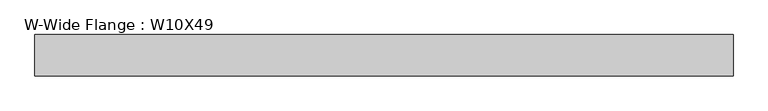
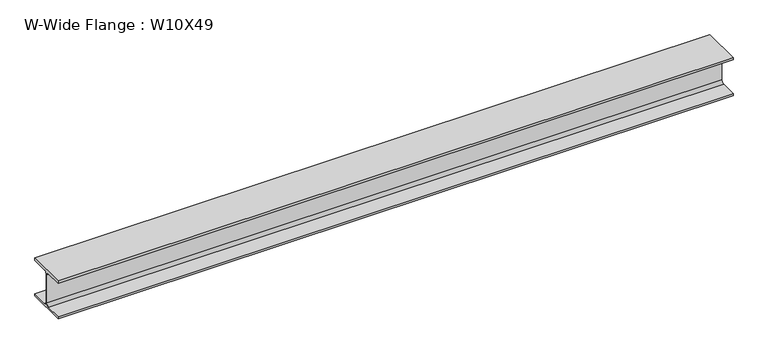
"""IFC4 building model written with IfcOpenShell, lengths in millimetres: beam geometry, W-Wide Flange : W10X49."""

from ifc_helpers import new_model, si_unit, point, frame, frame_2d, origin, place, context, project, spatial, polyline, circle_curve, trimmed, segment, composite_curve, outline, extrude, source, transform, mapped, element, save


def w_wide_flange_w10x49_85831f45(model_context):
    return source(origin(), model_context, "Body", "SweptSolid", [
        extrude(outline(composite_curve([segment(polyline([(127.0, -112.776), (127.0, -127.0), (-127.0, -127.0), (-127.0, -112.776), (-21.844, -112.776)]), True, "CONTINUOUS"), segment(trimmed(circle_curve(frame_2d((-21.844, -95.25)), 17.526), [point((-21.844, -112.776))], [point((-4.318, -95.25))], True, "CARTESIAN"), True, "CONTINUOUS"), segment(polyline([(-4.318, -95.25), (-4.318, 95.25)]), True, "CONTINUOUS"), segment(trimmed(circle_curve(frame_2d((-21.844, 95.25)), 17.526), [point((-4.318, 95.25))], [point((-21.844, 112.776))], True, "CARTESIAN"), True, "CONTINUOUS"), segment(polyline([(-21.844, 112.776), (-127.0, 112.776), (-127.0, 127.0), (127.0, 127.0), (127.0, 112.776), (21.844, 112.776)]), True, "CONTINUOUS"), segment(trimmed(circle_curve(frame_2d((21.844, 95.25)), 17.526), [point((21.844, 112.776))], [point((4.318, 95.25))], True, "CARTESIAN"), True, "CONTINUOUS"), segment(polyline([(4.318, 95.25), (4.318, -95.25)]), True, "CONTINUOUS"), segment(trimmed(circle_curve(frame_2d((21.844, -95.25)), 17.526), [point((4.318, -95.25))], [point((21.844, -112.776))], True, "CARTESIAN"), True, "CONTINUOUS"), segment(polyline([(21.844, -112.776), (127.0, -112.776)]), True, "CONTINUOUS")], self_intersect=False)), frame((-2142.7940989, 0.0, 0.0), z_axis=(1.0, 0.0, 0.0), x_axis=(0.0, 1.0, 0.0)), (0.0, 0.0, 1.0), 4286.3336069),
    ])


if __name__ == "__main__":
    model = new_model("IFC4")
    model_context = context("Model", 3, world=origin())
    ifc_project = project(units=[si_unit("LENGTHUNIT", "METRE", prefix="MILLI")], contexts=[model_context])
    site = spatial("IfcSite", under=ifc_project)
    building = spatial("IfcBuilding", under=site)
    placement = place(None, origin())
    w_wide_flange_w10x49_shape = w_wide_flange_w10x49_85831f45(model_context)
    element("IfcBeam", 1, ObjectType="W-Wide Flange : W10X49", at=placement, inside=building, context=model_context, shape_type="MappedRepresentation", body=[
        mapped(w_wide_flange_w10x49_shape, transform((0.0, 0.0, 0.0), x_axis=(1.0, 0.0, 0.0), y_axis=(0.0, 1.0, 0.0), z_axis=(0.0, 0.0, 1.0))),
    ])
    save(model, "model.ifc")

# Revit data of these elements
# Type "W-Wide Flange : W10X49"
#   Assembly Code = "B10"
#   W = 49
#   Length [instance default] = 1524 mm
#   bf = 254 mm
#   d = 254 mm
#   k = 31.75 mm
#   k2 = 17.526 mm
#   tf = 14.224 mm
#   tw = 8.636 mm
#   A = 0.0092903 m²
#   Structural Material [instance default] = Steel ASTM A992
# Element 1 (IfcBeam, "W-Wide Flange : W10X49")
#   Structural Material = Aluminum, Anodized Red
#   Materials on its faces: "Aluminum, Anodized Red"
# Materials
#   "Steel ASTM A992": class "Metal", colour RGB 128 0 0, transparency 0, Description = "Structural steel 50ksi", Cost = 0
#   "Aluminum, Anodized Red": class "Metal", colour RGB 120 120 120, transparency 0, Description = "Anodized aluminum, red", Cost = 0
